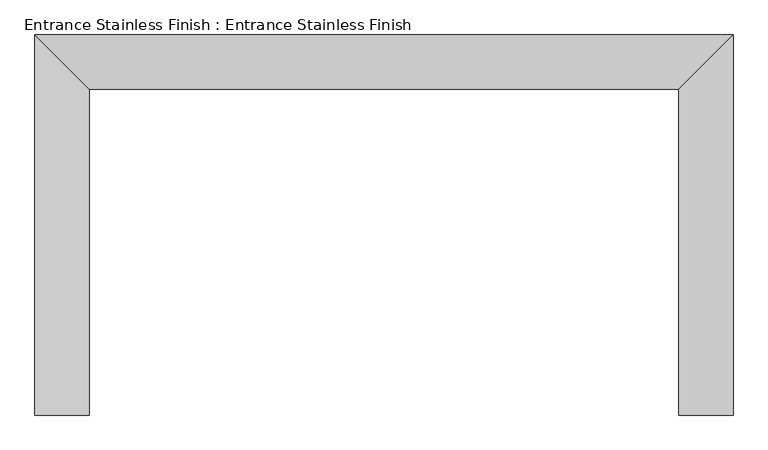
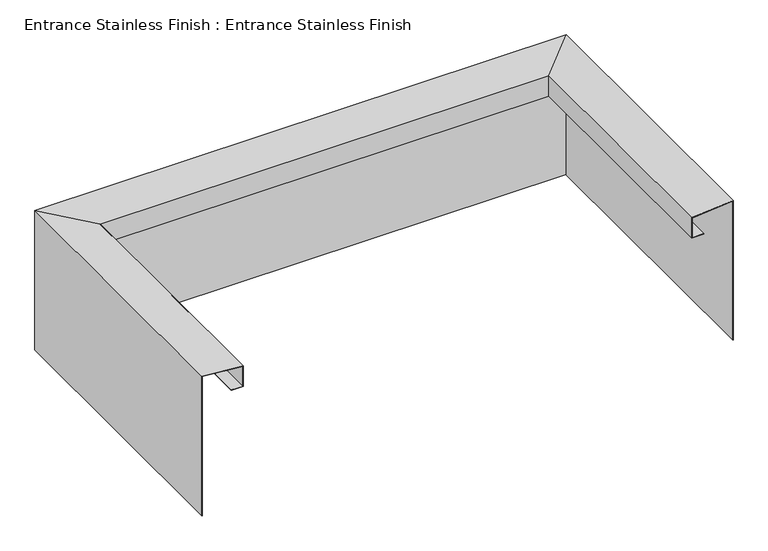
"""IFC4 building model written with IfcOpenShell, lengths in millimetres: proxy geometry, Entrance Stainless Finish : Entrance Stainless Finish."""

from ifc_helpers import new_model, si_unit, origin, place, context, project, spatial, faceted_brep, source, transform, mapped, element, save


def entrance_stainless_finish_entrance_stainless_finish_7ec3a08c(model_context):
    return source(origin(), model_context, "Body", "Brep", [
        faceted_brep([(26900.0, 300.0, 9737.5), (27000.0, 300.0, 9737.5), (27000.0, 300.0, 9740.5), (26903.0, 300.0, 9740.5), (26903.0, 300.0, 9917.2461426), (27247.0, 300.0, 9946.7318569), (27247.0, 300.0, 8700.0), (27250.0, 300.0, 8700.0), (27250.0, 300.0, 9950.0), (26900.0, 300.0, 9920.0), (26900.0, 2400.0, 9737.5), (23100.0, 2400.0, 9737.5), (23100.0, 300.0, 9737.5), (23000.0, 300.0, 9737.5), (23000.0, 2500.0, 9737.5), (27000.0, 2500.0, 9737.5), (27000.0, 2500.0, 9740.5), (23000.0, 2500.0, 9740.5), (23000.0, 300.0, 9740.5), (23097.0, 300.0, 9740.5), (23097.0, 2403.0, 9740.5), (26903.0, 2403.0, 9740.5), (26903.0, 2403.0, 9917.2461426), (27247.0, 2747.0, 9946.7318569), (27247.0, 2747.0, 8700.0), (22753.0, 2747.0, 8700.0), (22753.0, 300.0, 8700.0), (22750.0, 300.0, 8700.0), (22750.0, 2750.0, 8700.0), (27250.0, 2750.0, 8700.0), (27250.0, 2750.0, 9950.0), (26900.0, 2400.0, 9920.0), (23097.0, 2403.0, 9917.2461426), (22753.0, 2747.0, 9946.7318569), (22750.0, 2750.0, 9950.0), (23100.0, 2400.0, 9920.0), (23100.0, 300.0, 9920.0), (22750.0, 300.0, 9950.0), (22753.0, 300.0, 9946.7318569), (23097.0, 300.0, 9917.2461426)], [[[0, 1, 2, 3, 4, 5, 6, 7, 8, 9]], [[1, 0, 10, 11, 12, 13, 14, 15]], [[2, 1, 15, 16]], [[3, 2, 16, 17, 18, 19, 20, 21]], [[4, 3, 21, 22]], [[5, 4, 22, 23]], [[6, 5, 23, 24]], [[7, 6, 24, 25, 26, 27, 28, 29]], [[8, 7, 29, 30]], [[9, 8, 30, 31]], [[0, 9, 31, 10]], [[16, 15, 14, 17]], [[22, 21, 20, 32]], [[23, 22, 32, 33]], [[24, 23, 33, 25]], [[30, 29, 28, 34]], [[31, 30, 34, 35]], [[10, 31, 35, 11]], [[12, 36, 37, 27, 26, 38, 39, 19, 18, 13]], [[17, 14, 13, 18]], [[32, 20, 19, 39]], [[33, 32, 39, 38]], [[25, 33, 38, 26]], [[34, 28, 27, 37]], [[35, 34, 37, 36]], [[11, 35, 36, 12]]]),
    ])


if __name__ == "__main__":
    model = new_model("IFC4")
    model_context = context("Model", 3, world=origin())
    ifc_project = project(units=[si_unit("LENGTHUNIT", "METRE", prefix="MILLI")], contexts=[model_context])
    site = spatial("IfcSite", under=ifc_project)
    building = spatial("IfcBuilding", under=site)
    placement = place(None, origin())
    entrance_stainless_finish_entrance_stainless_finish_shape = entrance_stainless_finish_entrance_stainless_finish_7ec3a08c(model_context)
    element("IfcBuildingElementProxy", 1, Name="Entrance Stainless Finish : Entrance Stainless Finish", ObjectType="Entrance Stainless Finish : Entrance Stainless Finish", at=placement, inside=building, context=model_context, shape_type="MappedRepresentation", body=[
        mapped(entrance_stainless_finish_entrance_stainless_finish_shape, transform((0.0, 0.0, 0.0), x_axis=(1.0, 0.0, 0.0), y_axis=(0.0, 1.0, 0.0), z_axis=(0.0, 0.0, 1.0))),
    ])
    save(model, "model.ifc")

# Revit data of these elements
# Element 1 (IfcBuildingElementProxy, "Entrance Stainless Finish : Entrance Stainless Finish")
#   Materials on its faces: "00.Finish_Stainless Hairline"
# Materials
#   "00.Finish_Stainless Hairline": class "Generic", colour RGB 149 149 149, transparency 0, Description = "Acoustic ceiling tile", Cost = 0
